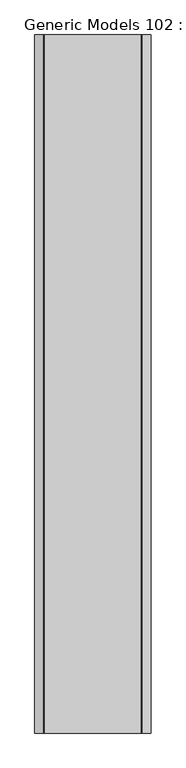
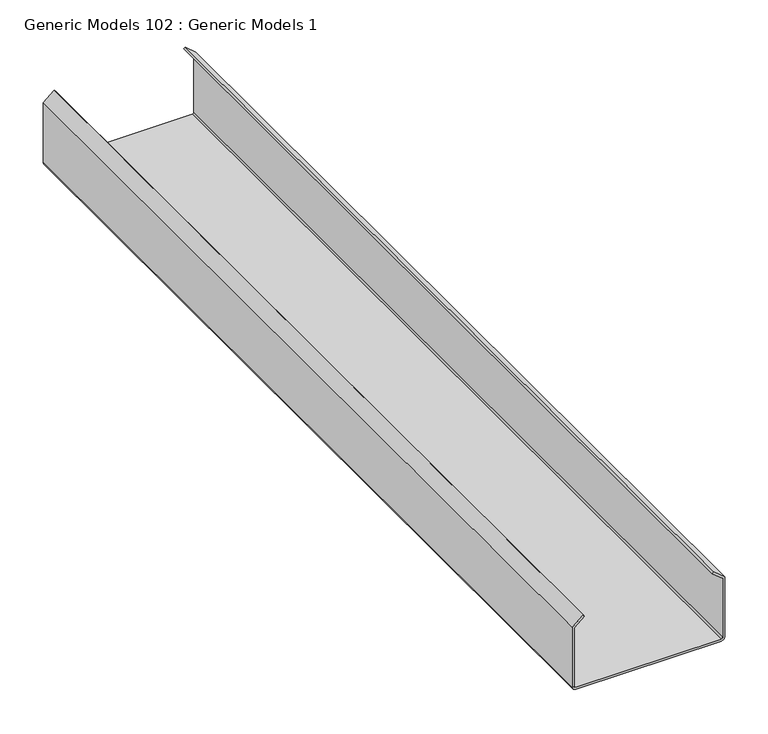
"""IFC4 building model written with IfcOpenShell, lengths in millimetres: proxy geometry, Generic Models 102 : Generic Models 1."""

import ifcopenshell
import ifcopenshell.guid

model = None  # the IFC model being written
_history = None  # IfcOwnerHistory: only IFC2X3 demands one
_inside = {}  # id of a spatial element -> (the spatial element, [elements in it])
_under = {}  # id of a project, library or spatial element -> (it, [spatial elements below it])
_declared = {}  # id of a project -> (the project, [libraries it declares])
_typed = {}  # id of a type object -> (the type object, [elements of that type])
_made_of = {}  # id of a material, layer set ... -> (it, [elements and type objects made of it])


def new_model(schema):
    """Start an empty IFC model of exactly this schema.

    Asked for "IFC4X3", IfcOpenShell would pick the latest addendum, in which some entities
    have other attributes; the version numbers below select the first issue.
    IFC2X3 requires an IfcOwnerHistory on every rooted entity: one is made here for all.
    """
    global model, _history
    if schema == "IFC4X3":
        model = ifcopenshell.file(schema_version=(4, 3, 0, 0))
    else:
        model = ifcopenshell.file(schema=schema)
    _inside.clear()
    _under.clear()
    _declared.clear()
    _typed.clear()
    _made_of.clear()
    _history = None
    if model.schema == "IFC2X3":
        org = make("IfcOrganization", Name="unknown")
        user = make(
            "IfcPersonAndOrganization",
            ThePerson=make("IfcPerson", FamilyName="unknown"),
            TheOrganization=org,
        )
        app = make(
            "IfcApplication",
            ApplicationDeveloper=org,
            Version="unknown",
            ApplicationFullName="unknown",
            ApplicationIdentifier="unknown",
        )
        _history = make(
            "IfcOwnerHistory",
            OwningUser=user,
            OwningApplication=app,
            ChangeAction="ADDED",
            CreationDate=0,
        )
    return model


def make(cls, **values):
    """One entity of the class cls with the attributes given. An attribute that is None is left unset."""
    return model.create_entity(
        cls, **{name: value for name, value in values.items() if value is not None}
    )


def rooted(cls, **values):
    """An entity with a GlobalId (a new one), such as an element, a storey or a relation."""
    return make(cls, GlobalId=ifcopenshell.guid.new(), OwnerHistory=_history, **values)


def si_unit(unit_type, name, prefix=None):
    """IfcSIUnit, for example si_unit("LENGTHUNIT", "METRE", prefix="MILLI")."""
    return make("IfcSIUnit", UnitType=unit_type, Prefix=prefix, Name=name)


def assignment(units):
    """IfcUnitAssignment: the units of a project."""
    return None if units is None else make("IfcUnitAssignment", Units=units)


def point(xyz):
    """IfcCartesianPoint."""
    return None if xyz is None else make("IfcCartesianPoint", Coordinates=xyz)


def direction(xyz):
    """IfcDirection."""
    return None if xyz is None else make("IfcDirection", DirectionRatios=xyz)


def frame(location, z_axis=None, x_axis=None):
    """IfcAxis2Placement3D, a coordinate frame: its origin and axes. An axis left out is left unset."""
    return make(
        "IfcAxis2Placement3D",
        Location=point(location),
        Axis=direction(z_axis),
        RefDirection=direction(x_axis),
    )


def frame_2d(location, x_axis=None):
    """IfcAxis2Placement2D, a coordinate frame in the plane: its origin and x axis."""
    return make(
        "IfcAxis2Placement2D", Location=point(location), RefDirection=direction(x_axis)
    )


def origin():
    """The frame at (0, 0, 0) with its axes left unset."""
    return frame((0.0, 0.0, 0.0))


def place(relative_to, where):
    """IfcLocalPlacement: puts the frame where relative to a parent placement (None: the world)."""
    return make(
        "IfcLocalPlacement", PlacementRelTo=relative_to, RelativePlacement=where
    )


def context(
    kind, dimensions, precision=None, world=None, true_north=None, identifier=None
):
    """IfcGeometricRepresentationContext, for example the 3D "Model" context."""
    return make(
        "IfcGeometricRepresentationContext",
        ContextIdentifier=identifier,
        ContextType=kind,
        CoordinateSpaceDimension=dimensions,
        Precision=precision,
        WorldCoordinateSystem=world,
        TrueNorth=true_north,
    )


def project(units=None, contexts=None):
    """IfcProject with its units and contexts."""
    return rooted(
        "IfcProject",
        Name="project",
        RepresentationContexts=contexts,
        UnitsInContext=assignment(units),
    )


def spatial(cls, under=None, at=None, **own):
    """A site, building, storey or space (cls), placed at a placement, below another one or the project."""
    s = rooted(cls, ObjectPlacement=at, **own)
    if under is not None:
        _under.setdefault(under.id(), (under, []))[1].append(s)
    return s


def polyline(points):
    """IfcPolyline through the points."""
    return make("IfcPolyline", Points=[point(p) for p in points])


def circle_curve(where, radius):
    """IfcCircle in the frame where."""
    return make("IfcCircle", Position=where, Radius=radius)


def trimmed(basis, trim1, trim2, sense, master):
    """IfcTrimmedCurve: the piece of a basis curve between two trims."""
    return make(
        "IfcTrimmedCurve",
        BasisCurve=basis,
        Trim1=trim1,
        Trim2=trim2,
        SenseAgreement=sense,
        MasterRepresentation=master,
    )


def segment(curve, same_sense, transition):
    """IfcCompositeCurveSegment."""
    return make(
        "IfcCompositeCurveSegment",
        Transition=transition,
        SameSense=same_sense,
        ParentCurve=curve,
    )


def composite_curve(segments, self_intersect=None):
    """IfcCompositeCurve: segments joined end to end."""
    return make("IfcCompositeCurve", Segments=segments, SelfIntersect=self_intersect)


def outline(outer, holes=None, kind="AREA"):
    """IfcArbitraryClosedProfileDef: a profile drawn as a closed curve; with holes, ...WithVoids."""
    if holes is None:
        return make("IfcArbitraryClosedProfileDef", ProfileType=kind, OuterCurve=outer)
    return make(
        "IfcArbitraryProfileDefWithVoids",
        ProfileType=kind,
        OuterCurve=outer,
        InnerCurves=holes,
    )


def extrude(swept, where, along, depth):
    """IfcExtrudedAreaSolid: the profile swept, set in the frame where, extruded along a direction by depth."""
    return make(
        "IfcExtrudedAreaSolid",
        SweptArea=swept,
        Position=where,
        ExtrudedDirection=direction(along),
        Depth=depth,
    )


def shape(context_of_items, identifier, shape_type, items):
    """IfcShapeRepresentation: the items that make up one representation, for example the "Body"."""
    return make(
        "IfcShapeRepresentation",
        ContextOfItems=context_of_items,
        RepresentationIdentifier=identifier,
        RepresentationType=shape_type,
        Items=items,
    )


def source(mapping_origin, context_of_items, identifier, shape_type, items):
    """IfcRepresentationMap: a shape defined once, which mapped items show again and again."""
    return make(
        "IfcRepresentationMap",
        MappingOrigin=mapping_origin,
        MappedRepresentation=shape(context_of_items, identifier, shape_type, items),
    )


def transform(
    local_origin,
    x_axis=None,
    y_axis=None,
    z_axis=None,
    scale=None,
    scale2=None,
    scale3=None,
    uniform=True,
):
    """IfcCartesianTransformationOperator3D, or its non-uniform kind. x_axis, y_axis, z_axis: its Axis1, 2, 3."""
    if uniform:
        return make(
            "IfcCartesianTransformationOperator3D",
            Axis1=direction(x_axis),
            Axis2=direction(y_axis),
            LocalOrigin=point(local_origin),
            Scale=scale,
            Axis3=direction(z_axis),
        )
    return make(
        "IfcCartesianTransformationOperator3DnonUniform",
        Axis1=direction(x_axis),
        Axis2=direction(y_axis),
        LocalOrigin=point(local_origin),
        Scale=scale,
        Axis3=direction(z_axis),
        Scale2=scale2,
        Scale3=scale3,
    )


def mapped(mapping_source, mapping_target):
    """IfcMappedItem: shows the shape of a source again, moved by a transform."""
    return make(
        "IfcMappedItem", MappingSource=mapping_source, MappingTarget=mapping_target
    )


def made_of(thing, what):
    """Note that an element or type object is made of a material, layer set ...; save() writes the relation."""
    if what is not None:
        _made_of.setdefault(what.id(), (what, []))[1].append(thing)
    return thing


def element(
    cls,
    number,
    at=None,
    inside=None,
    cuts=None,
    type_object=None,
    material=None,
    context=None,
    identifier="Body",
    shape_type=None,
    held_by="IfcProductDefinitionShape",
    body=None,
    shapes=None,
    **own,
):
    """One element of the class cls, such as IfcWall. Its Tag is "e" and its number.

    at: its placement. inside: the storey or other place that contains it. cuts: it is an
    opening in that element (IfcRelVoidsElement). A single representation is given by context,
    identifier, shape_type and body (its items); several are given by shapes. held_by: the class
    of the entity that holds the representations. save() writes the other relations.
    """
    e = rooted(cls, Tag="e%d" % number, ObjectPlacement=at, **own)
    if body is not None:
        shapes = [shape(context, identifier, shape_type, body)]
    if shapes is not None:
        e.Representation = make(held_by, Representations=shapes)
    if inside is not None:
        _inside.setdefault(inside.id(), (inside, []))[1].append(e)
    if cuts is not None:
        rooted(
            "IfcRelVoidsElement", RelatingBuildingElement=cuts, RelatedOpeningElement=e
        )
    if type_object is not None:
        _typed.setdefault(type_object.id(), (type_object, []))[1].append(e)
    return made_of(e, material)


def aggregate(whole, parts):
    """IfcRelAggregates: a whole, such as a stair, and the parts it consists of."""
    return rooted("IfcRelAggregates", RelatingObject=whole, RelatedObjects=parts)


def save(model, path):
    """Write the relations noted so far, then the file.

    IfcRelAggregates (storeys below a building ...), IfcRelContainedInSpatialStructure (elements
    in a storey), IfcRelDefinesByType, IfcRelAssociatesMaterial and IfcRelDeclares: one each for
    every whole, place, type object, material and project.
    """
    for whole, parts in _under.values():
        aggregate(whole, parts)
    for where, things in _inside.values():
        rooted(
            "IfcRelContainedInSpatialStructure",
            RelatedElements=things,
            RelatingStructure=where,
        )
    for kind, things in _typed.values():
        rooted("IfcRelDefinesByType", RelatedObjects=things, RelatingType=kind)
    for what, things in _made_of.values():
        rooted("IfcRelAssociatesMaterial", RelatedObjects=things, RelatingMaterial=what)
    for by, libraries in _declared.values():
        rooted("IfcRelDeclares", RelatingContext=by, RelatedDefinitions=libraries)
    model.write(path)


def generic_models_102_generic_models_1_8a2dd616(model_context):
    return source(origin(), model_context, "Body", "SweptSolid", [
        extrude(outline(composite_curve([segment(polyline([(4498.578125, 52222.4), (4510.823229, 52207.8068534), (4508.6950617, 52206.021109), (4497.282664, 52219.621875), (4414.3677682, 52219.621875)]), True, "CONTINUOUS"), segment(trimmed(circle_curve(frame_2d((4414.4412941, 52217.6381931)), 1.9850441), [point((4414.3677682, 52219.621875))], [point((4412.45625, 52217.6381931))], True, "CARTESIAN"), True, "CONTINUOUS"), segment(polyline([(4412.45625, 52217.6381931), (4412.45625, 52023.9610661)]), True, "CONTINUOUS"), segment(trimmed(circle_curve(frame_2d((4414.4419899, 52023.9610661)), 1.9857399), [point((4412.45625, 52023.9610661))], [point((4414.3365981, 52021.978125))], True, "CARTESIAN"), True, "CONTINUOUS"), segment(polyline([(4414.3365981, 52021.978125), (4497.282664, 52021.978125), (4508.718285, 52035.6065673), (4510.8464522, 52033.820823), (4498.578125, 52019.2), (4414.440625, 52019.2)]), True, "CONTINUOUS"), segment(trimmed(circle_curve(frame_2d((4414.440625, 52023.9625)), 4.7625), [point((4414.440625, 52019.2))], [point((4409.678125, 52023.9625))], False, "CARTESIAN"), True, "CONTINUOUS"), segment(polyline([(4409.678125, 52023.9625), (4409.678125, 52217.6375)]), True, "CONTINUOUS"), segment(trimmed(circle_curve(frame_2d((4414.440625, 52217.6375)), 4.7625), [point((4409.678125, 52217.6375))], [point((4414.440625, 52222.4))], False, "CARTESIAN"), True, "CONTINUOUS"), segment(polyline([(4414.440625, 52222.4), (4498.578125, 52222.4)]), True, "CONTINUOUS")], self_intersect=False)), frame((0.0, 0.0, 0.0), z_axis=(0.0, 1.0, 0.0), x_axis=(0.0, 0.0, 1.0)), (0.0, 0.0, 1.0), 1219.2),
    ])


if __name__ == "__main__":
    model = new_model("IFC4")
    model_context = context("Model", 3, world=origin())
    ifc_project = project(units=[si_unit("LENGTHUNIT", "METRE", prefix="MILLI")], contexts=[model_context])
    site = spatial("IfcSite", under=ifc_project)
    building = spatial("IfcBuilding", under=site)
    placement = place(None, origin())
    generic_models_102_generic_models_1_shape = generic_models_102_generic_models_1_8a2dd616(model_context)
    element("IfcBuildingElementProxy", 1, Name="Generic Models 102 : Generic Models 1", ObjectType="Generic Models 102 : Generic Models 1", at=placement, inside=building, context=model_context, shape_type="MappedRepresentation", body=[
        mapped(generic_models_102_generic_models_1_shape, transform((0.0, 0.0, 0.0), x_axis=(1.0, 0.0, 0.0), y_axis=(0.0, 1.0, 0.0), z_axis=(0.0, 0.0, 1.0))),
    ])
    save(model, "model.ifc")

# Revit data of these elements
# Element 1 (IfcBuildingElementProxy, "Generic Models 102 : Generic Models 1")
#   Materials on its faces: "EXISTING GIRT"
# Materials
#   "EXISTING GIRT": class "Metal", colour RGB 199 199 199, transparency 0, Description = "Carbon steel", Cost = 0
